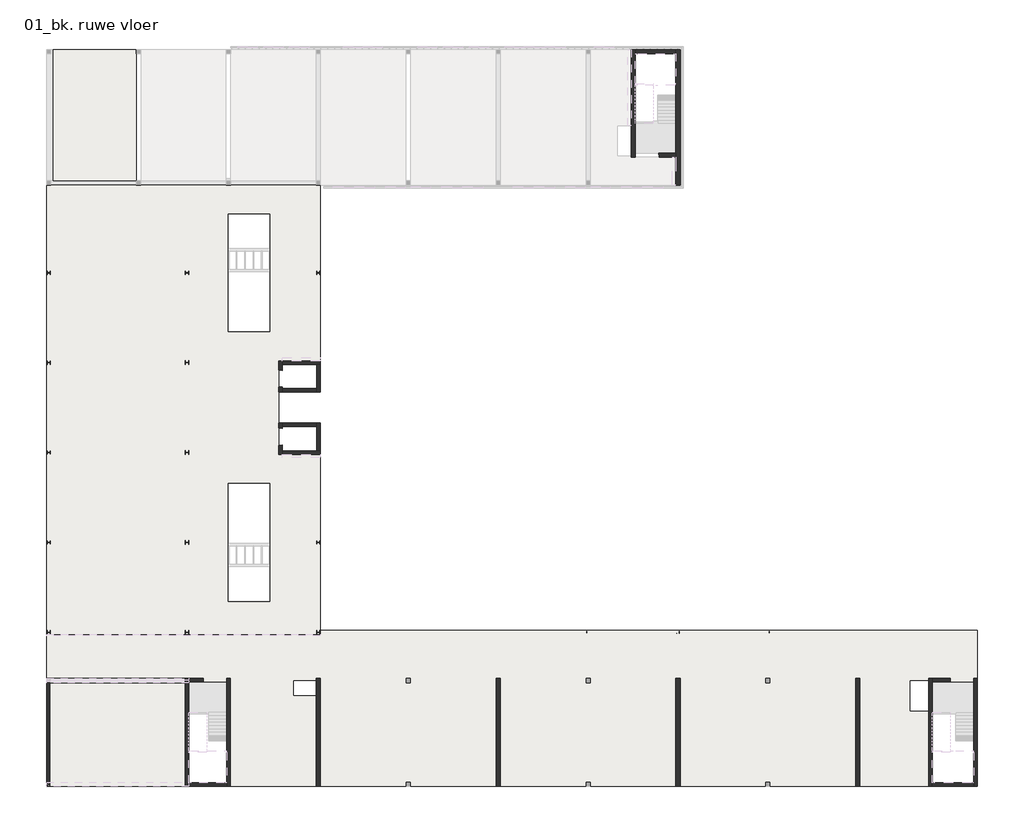
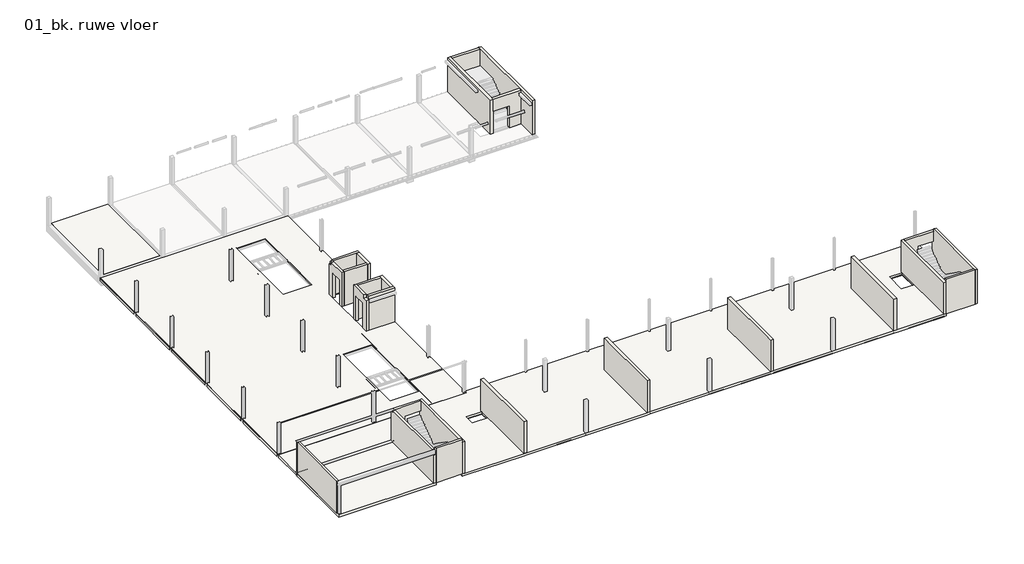
# One storey, part 1 of 4: 25 walls, 20 slabs.
# Revit data of these elements (continued)
# Type "NLRS_21_WA_beton ihw 250_gen_rsf"
#   Keynote = ""
#   Type IfcGUID = "1pBmRfcsbA7BE9s_rekBP3"
#   Description = "buitenwand beton ihw, generiek"
#   Assembly Code = "21.21"
#   IfcExportAs = "IfcWall"
#   Layers, outside or top first: 250 mm "NLRS_f2_beton ihwg_gen_rsf" (function 1)
# Type "NLRS_21_WA_kalkzandsteen CS12 214_gen_rsf"
#   Keynote = ""
#   Type IfcGUID = "2$hNzCXOT3YR8V$0Cfyzq0"
#   Type Comments = "blokken/elementen gelijmd, d =214mm"
#   Description = "dragende buitenwand kalkzandsteen, klasse CS12"
#   Assembly Code = "21.21"
#   IfcExportAs = "IfcWall"
#   Layers, outside or top first: 214 mm "NLRS_f1_kalkzandsteen_gen_rsf" (function 1)
# Type "NLRS_22_WA_beton prefab 300_gen_rsf"
#   Keynote = ""
#   Type IfcGUID = "2ajLwCSRTE_9I1Spg4sCRo"
#   Description = "binnenwand beton prefab, generiek"
#   Assembly Code = "22.21"
#   IfcExportAs = "IfcWall"
#   Layers, outside or top first: 300 mm "NLRS_f2_beton prefab_gen_rsf" (function 1)
# Type "NLRS_21_WA_beton prefab 300_gen_rsf"
#   Keynote = ""
#   Type IfcGUID = "2ajLwCSRTE_9I1Spg4sCru"
#   Description = "buitenwand beton prefab, generiek"
#   Assembly Code = "21.21"
#   IfcExportAs = "IfcWall"
#   Layers, outside or top first: 300 mm "NLRS_f2_beton prefab_gen_rsf" (function 1)
# Type "NLRS_22_WA_beton prefab 250_gen_rsf"
#   Keynote = ""
#   Type IfcGUID = "2GRbcre991teoKeCLB8LsU"
#   Description = "binnenwand beton prefab, generiek"
#   Assembly Code = "22.21"
#   IfcExportAs = "IfcWall"
#   Layers, outside or top first: 250 mm "NLRS_f2_beton prefab_gen_rsf" (function 1)
# Type "NLRS_21_WA_beton prefab 250_gen_rsf"
#   Keynote = ""
#   Type IfcGUID = "3N5NK1g7D9AwpiDnyE93lX"
#   Description = "buitenwand beton prefab, generiek"
#   Assembly Code = "21.21"
#   IfcExportAs = "IfcWall"
#   Layers, outside or top first: 250 mm "NLRS_f2_beton prefab_gen_rsf" (function 1)
# Element 1 (IfcSlab, "NLRS_23_FL_breedplaat 260_gen_rsf")
#   IfcGUID = "2ajLwCSRTE_9I1Spg4tpLw"
#   Comments = ""
#   Height Offset From Level = 0 mm
#   built-in parameter 1001954 = 1
#   IsExternal = no
#   LoadBearing = yes
#   Phase Created = NLRS_nieuw
#   Materials on its faces: "NLRS_f2_beton ihwg_gen_rsf"
# Element 2 (IfcSlab, "NLRS_23_FL_breedplaat 260_gen_rsf")
#   IfcGUID = "3_OCAr9yj6mwah3L5tr_i6"
#   Height Offset From Level = 0 mm
#   built-in parameter 1001954 = 1
#   IsExternal = no
#   LoadBearing = yes
#   Phase Created = NLRS_nieuw
#   Materials on its faces: "NLRS_f2_beton ihwg_gen_rsf"
# Element 3 (IfcSlab, "NLRS_23_FL_druklaag 70_gen_rsf")
#   IfcGUID = "2GRbcre991teoKeCLB8MGT"
#   Height Offset From Level = 0 mm
#   built-in parameter 1001954 = 1
#   IsExternal = no
#   LoadBearing = yes
#   Phase Created = NLRS_nieuw
#   Materials on its faces: "NLRS_f2_beton ihwg_gen_rsf"
# Element 4 (IfcSlab, "NLRS_23_FL_kanaalplaat 260_gen_rsf")
#   IfcGUID = "0zo1UjqZ91lRsfCKsOObA6"
#   built-in parameter 1001955 = -1.5708 (stored number, unit not read)
#   Height Offset From Level = -70 mm
#   built-in parameter 1001954 = 1
#   IsExternal = no
#   LoadBearing = yes
#   Phase Created = NLRS_nieuw
#   Materials on its faces: "NLRS_f2_beton prefab_gen_rsf"
# Element 5 (IfcSlab, "NLRS_23_FL_kanaalplaat 260_gen_rsf")
#   IfcGUID = "0zo1UjqZ91lRsfCKsOObtg"
#   built-in parameter 1001955 = -1.5708 (stored number, unit not read)
#   Height Offset From Level = -70 mm
#   built-in parameter 1001954 = 1
#   IsExternal = no
#   LoadBearing = yes
#   Phase Created = NLRS_nieuw
#   Materials on its faces: "NLRS_f2_beton prefab_gen_rsf"
# Element 6 (IfcSlab, "NLRS_23_FL_kanaalplaat 260_gen_rsf")
#   IfcGUID = "0zo1UjqZ91lRsfCKsOObzx"
#   built-in parameter 1001955 = -1.5708 (stored number, unit not read)
#   Height Offset From Level = -70 mm
#   built-in parameter 1001954 = 1
#   IsExternal = no
#   LoadBearing = yes
#   Phase Created = NLRS_nieuw
#   Materials on its faces: "NLRS_f2_beton prefab_gen_rsf"
# Element 7 (IfcSlab, "NLRS_23_FL_kanaalplaat 260_gen_rsf")
#   IfcGUID = "0OswKhMc1Dju7i6LqsClK9"
#   built-in parameter 1001955 = -1.5708 (stored number, unit not read)
#   Height Offset From Level = -70 mm
#   built-in parameter 1001954 = 1
#   IsExternal = no
#   LoadBearing = yes
#   Phase Created = NLRS_nieuw
#   Materials on its faces: "NLRS_f2_beton prefab_gen_rsf"
# Element 8 (IfcSlab, "NLRS_23_FL_kanaalplaat 260_gen_rsf")
#   IfcGUID = "0OswKhMc1Dju7i6LqsClM0"
#   built-in parameter 1001955 = 1.5708 (stored number, unit not read)
#   Height Offset From Level = -70 mm
#   built-in parameter 1001954 = 1
#   IsExternal = no
#   LoadBearing = yes
#   Phase Created = NLRS_nieuw
#   Materials on its faces: "NLRS_f2_beton prefab_gen_rsf"
# Element 9 (IfcSlab, "NLRS_23_FL_kanaalplaat 260_gen_rsf")
#   IfcGUID = "0OswKhMc1Dju7i6LqsClMb"
#   Height Offset From Level = -70 mm
#   built-in parameter 1001954 = 1
#   IsExternal = no
#   LoadBearing = yes
#   Phase Created = NLRS_nieuw
#   Materials on its faces: "NLRS_f2_beton prefab_gen_rsf"
# Element 10 (IfcSlab, "NLRS_23_FL_kanaalplaat 260_gen_rsf")
#   IfcGUID = "0OswKhMc1Dju7i6LqsClTA"
#   built-in parameter 1001955 = -1.5708 (stored number, unit not read)
#   Height Offset From Level = -70 mm
#   built-in parameter 1001954 = 1
#   IsExternal = no
#   LoadBearing = yes
#   Phase Created = NLRS_nieuw
#   Materials on its faces: "NLRS_f2_beton prefab_gen_rsf"
# Element 11 (IfcSlab, "NLRS_23_FL_kanaalplaat 260_gen_rsf")
#   IfcGUID = "0OswKhMc1Dju7i6LqsCl1Q"
#   built-in parameter 1001955 = 1.5708 (stored number, unit not read)
#   Height Offset From Level = -70 mm
#   built-in parameter 1001954 = 1
#   IsExternal = no
#   LoadBearing = yes
#   Phase Created = NLRS_nieuw
#   Materials on its faces: "NLRS_f2_beton prefab_gen_rsf"
# Element 12 (IfcSlab, "NLRS_23_FL_kanaalplaat 260_gen_rsf")
#   IfcGUID = "0OswKhMc1Dju7i6LqsCl1J"
#   built-in parameter 1001955 = 1.5708 (stored number, unit not read)
#   Height Offset From Level = -70 mm
#   built-in parameter 1001954 = 1
#   IsExternal = no
#   LoadBearing = yes
#   Phase Created = NLRS_nieuw
#   Materials on its faces: "NLRS_f2_beton prefab_gen_rsf"
# Element 13 (IfcSlab, "NLRS_23_FL_kanaalplaat 260_gen_rsf")
#   IfcGUID = "0OswKhMc1Dju7i6LqsCl1k"
#   built-in parameter 1001955 = 1.5708 (stored number, unit not read)
#   Height Offset From Level = -70 mm
#   built-in parameter 1001954 = 1
#   IsExternal = no
#   LoadBearing = yes
#   Phase Created = NLRS_nieuw
#   Materials on its faces: "NLRS_f2_beton prefab_gen_rsf"
# Element 14 (IfcSlab, "NLRS_23_FL_kanaalplaat 260_gen_rsf")
#   IfcGUID = "0OswKhMc1Dju7i6LqsCl1d"
#   built-in parameter 1001955 = -1.5708 (stored number, unit not read)
#   Height Offset From Level = -70 mm
#   built-in parameter 1001954 = 1
#   IsExternal = no
#   LoadBearing = yes
#   Phase Created = NLRS_nieuw
#   Materials on its faces: "NLRS_f2_beton prefab_gen_rsf"
# Element 15 (IfcSlab, "NLRS_23_FL_kanaalplaat 260_gen_rsf")
#   IfcGUID = "0OswKhMc1Dju7i6LqsCl1m"
#   Height Offset From Level = -70 mm
#   built-in parameter 1001954 = 1
#   IsExternal = no
#   LoadBearing = yes
#   Phase Created = NLRS_nieuw
#   Materials on its faces: "NLRS_f2_beton prefab_gen_rsf"
# Element 16 (IfcSlab, "NLRS_23_FL_kanaalplaat 260_gen_rsf")
#   IfcGUID = "0OswKhMc1Dju7i6LqsCl2B"
#   built-in parameter 1001955 = 1.5708 (stored number, unit not read)
#   Height Offset From Level = -70 mm
#   built-in parameter 1001954 = 1
#   IsExternal = no
#   LoadBearing = yes
#   Phase Created = NLRS_nieuw
#   Materials on its faces: "NLRS_f2_beton prefab_gen_rsf"
# Element 17 (IfcSlab, "NLRS_23_FL_breedplaat 260_gen_rsf")
#   IfcGUID = "3aMdMHoe12P9KDGPyaIhcT"
#   built-in parameter 1001955 = 1.5708 (stored number, unit not read)
#   Height Offset From Level = 0 mm
#   built-in parameter 1001954 = 1
#   IsExternal = no
#   LoadBearing = yes
#   Phase Created = NLRS_nieuw
#   Materials on its faces: "NLRS_f2_beton ihwg_gen_rsf"
# Element 18 (IfcSlab, "NLRS_23_FL_breedplaat schil 60_gen_rsf")
#   IfcGUID = "2hjDq_lp57$vrUvPCETdlA"
#   Comments = ""
#   built-in parameter 1001955 = -1.5708 (stored number, unit not read)
#   Height Offset From Level = -200 mm
#   built-in parameter 1001954 = 1
#   IsExternal = no
#   LoadBearing = yes
#   Phase Created = NLRS_nieuw
#   Materials on its faces: "NLRS_f2_beton prefab_gen_rsf"
# Element 19 (IfcSlab, "NLRS_23_FL_breedplaat schil 60_gen_rsf")
#   IfcGUID = "2hjDq_lp57$vrUvPCETOIZ"
#   Comments = ""
#   built-in parameter 1001955 = -1.5708 (stored number, unit not read)
#   Height Offset From Level = -200 mm
#   built-in parameter 1001954 = 1
#   IsExternal = no
#   LoadBearing = yes
#   Phase Created = NLRS_nieuw
#   Materials on its faces: "NLRS_f2_beton prefab_gen_rsf"
# Element 20 (IfcSlab, "NLRS_23_FL_breedplaat schil 60_gen_rsf")
#   IfcGUID = "1q3Kx8wcTFnf_3PJz4ij95"
#   Comments = ""
#   Height Offset From Level = -200 mm
#   built-in parameter 1001954 = 1
#   IsExternal = no
#   LoadBearing = yes
#   Phase Created = NLRS_nieuw
#   Materials on its faces: "NLRS_f2_beton prefab_gen_rsf"
# Element 21 (IfcWall, "NLRS_22_WA_beton ihw 250_gen_rsf")
#   IfcGUID = "13lTCcCQ95UOWcvnmPh7qn"
#   Comments = ""
#   Top Offset = 0 mm
#   Base Offset = 0 mm
#   wall height = 3540 mm
#   IsExternal = no
#   LoadBearing = yes
#   Phase Created = NLRS_nieuw
#   Base Constraint = 01_bk. ruwe vloer
#   Top Constraint = 02_ok ruwe vloer
#   Materials on its faces: "NLRS_f2_beton ihwg_gen_rsf"
# Element 22 (IfcWall, "NLRS_22_WA_beton ihw 250_gen_rsf")
#   IfcGUID = "13lTCcCQ95UOWcvnmPh7qi"
#   Comments = ""
#   Top Offset = 0 mm
#   Base Offset = 0 mm
#   wall height = 3540 mm
#   IsExternal = no
#   LoadBearing = yes
#   Phase Created = NLRS_nieuw
#   Base Constraint = 01_bk. ruwe vloer
#   Top Constraint = 02_ok ruwe vloer
#   Materials on its faces: "NLRS_f2_beton ihwg_gen_rsf"
# Element 23 (IfcWall, "NLRS_22_WA_beton ihw 300_gen_rsf")
#   IfcGUID = "13lTCcCQ95UOWcvnmPh7qk"
#   Comments = ""
#   Top Offset = 0 mm
#   Base Offset = 0 mm
#   wall height = 3540 mm
#   IsExternal = no
#   LoadBearing = yes
#   Phase Created = NLRS_nieuw
#   Base Constraint = 01_bk. ruwe vloer
#   Top Constraint = 02_ok ruwe vloer
#   Materials on its faces: "NLRS_f2_beton ihwg_gen_rsf"
# Element 24 (IfcWall, "NLRS_22_WA_beton ihw 300_gen_rsf")
#   IfcGUID = "13lTCcCQ95UOWcvnmPh7qg"
#   Comments = ""
#   Top Offset = 0 mm
#   Base Offset = 0 mm
#   wall height = 3540 mm
#   IsExternal = no
#   LoadBearing = yes
#   Phase Created = NLRS_nieuw
#   Base Constraint = 01_bk. ruwe vloer
#   Top Constraint = 02_ok ruwe vloer
#   Materials on its faces: "NLRS_f2_beton ihwg_gen_rsf"
# Element 25 (IfcWall, "NLRS_22_WA_beton ihw 300_gen_rsf")
#   IfcGUID = "13lTCcCQ95UOWcvnmPh7qc"
#   Comments = ""
#   Top Offset = 0 mm
#   Base Offset = 0 mm
#   wall height = 3540 mm
#   IsExternal = no
#   LoadBearing = yes
#   Phase Created = NLRS_nieuw
#   Base Constraint = 01_bk. ruwe vloer
#   Top Constraint = 02_ok ruwe vloer
#   Materials on its faces: "NLRS_f2_beton ihwg_gen_rsf"
# Element 26 (IfcWall, "NLRS_22_WA_beton ihw 300_gen_rsf")
#   IfcGUID = "13lTCcCQ95UOWcvnmPh7qY"
#   Comments = ""
#   Top Offset = 0 mm
#   Base Offset = 0 mm
#   wall height = 3540 mm
#   IsExternal = no
#   LoadBearing = yes
#   Phase Created = NLRS_nieuw
#   Base Constraint = 01_bk. ruwe vloer
#   Top Constraint = 02_ok ruwe vloer
#   Materials on its faces: "NLRS_f2_beton ihwg_gen_rsf"
# Element 27 (IfcWall, "NLRS_21_WA_beton ihw 250_gen_rsf")
#   IfcGUID = "13lTCcCQ95UOWcvnmPh7rS"
#   Comments = ""
#   Top Offset = 0 mm
#   Base Offset = 0 mm
#   wall height = 3800 mm
#   IsExternal = yes
#   LoadBearing = yes
#   Phase Created = NLRS_nieuw
#   Base Constraint = 01_bk. ruwe vloer
#   Top Constraint = 02_bk ruwe vloer
#   Materials on its faces: "NLRS_f2_beton ihwg_gen_rsf"
# Element 28 (IfcWall, "NLRS_21_WA_kalkzandsteen CS12 214_gen_rsf")
#   IfcGUID = "13lTCcCQ95UOWcvnmPh7rU"
#   Comments = ""
#   Top Offset = 0 mm
#   Base Offset = 0 mm
#   wall height = 3540 mm
#   IsExternal = yes
#   LoadBearing = yes
#   Phase Created = NLRS_nieuw
#   Base Constraint = 01_bk. ruwe vloer
#   Top Constraint = 02_ok ruwe vloer
#   Materials on its faces: "NLRS_f1_kalkzandsteen_gen_rsf"
# Element 29 (IfcWall, "NLRS_21_WA_beton ihw 250_gen_rsf")
#   IfcGUID = "13lTCcCQ95UOWcvnmPh7rO"
#   Top Offset = 0 mm
#   Base Offset = 0 mm
#   wall height = 3800 mm
#   IsExternal = yes
#   LoadBearing = yes
#   Phase Created = NLRS_nieuw
#   Base Constraint = 01_bk. ruwe vloer
#   Top Constraint = 02_bk ruwe vloer
#   Materials on its faces: "NLRS_f2_beton ihwg_gen_rsf"
# Element 30 (IfcWall, "NLRS_22_WA_beton ihw 250_gen_rsf")
#   IfcGUID = "13lTCcCQ95UOWcvnmPh7rQ"
#   Top Offset = 0 mm
#   Base Offset = 0 mm
#   wall height = 3540 mm
#   IsExternal = no
#   LoadBearing = yes
#   Phase Created = NLRS_nieuw
#   Base Constraint = 01_bk. ruwe vloer
#   Top Constraint = 02_ok ruwe vloer
#   Materials on its faces: "NLRS_f2_beton ihwg_gen_rsf"
# Element 31 (IfcWall, "NLRS_22_WA_beton ihw 250_gen_rsf")
#   IfcGUID = "13lTCcCQ95UOWcvnmPh7rK"
#   Comments = ""
#   Top Offset = 0 mm
#   Base Offset = 0 mm
#   wall height = 3540 mm
#   IsExternal = no
#   LoadBearing = yes
#   Phase Created = NLRS_nieuw
#   Base Constraint = 01_bk. ruwe vloer
#   Top Constraint = 02_ok ruwe vloer
#   Materials on its faces: "NLRS_f2_beton ihwg_gen_rsf"
# Element 32 (IfcWall, "NLRS_21_WA_beton ihw 250_gen_rsf")
#   IfcGUID = "13lTCcCQ95UOWcvnmPh7rM"
#   Top Offset = 0 mm
#   Base Offset = 0 mm
#   wall height = 3800 mm
#   IsExternal = yes
#   LoadBearing = yes
#   Phase Created = NLRS_nieuw
#   Base Constraint = 01_bk. ruwe vloer
#   Top Constraint = 02_bk ruwe vloer
#   Materials on its faces: "NLRS_f2_beton ihwg_gen_rsf"
# Element 33 (IfcWall, "NLRS_22_WA_beton ihw 250_gen_rsf")
#   IfcGUID = "13lTCcCQ95UOWcvnmPh7rG"
#   Top Offset = 0 mm
#   Base Offset = 0 mm
#   wall height = 3540 mm
#   IsExternal = no
#   LoadBearing = yes
#   Phase Created = NLRS_nieuw
#   Base Constraint = 01_bk. ruwe vloer
#   Top Constraint = 02_ok ruwe vloer
#   Materials on its faces: "NLRS_f2_beton ihwg_gen_rsf"
# Element 34 (IfcWall, "NLRS_22_WA_beton prefab 300_gen_rsf")
#   IfcGUID = "13lTCcCQ95UOWcvnmPh7s_"
#   Comments = ""
#   built-in parameter 1001111 = 20 mm
#   Top Offset = 0 mm
#   Base Offset = 20 mm
#   wall height = 3780 mm
#   IsExternal = no
#   LoadBearing = yes
#   Phase Created = NLRS_nieuw
#   Base Constraint = 01_bk. ruwe vloer
#   Top Constraint = 02_bk ruwe vloer
#   Materials on its faces: "NLRS_f2_beton prefab_gen_rsf"
# Element 35 (IfcWall, "NLRS_21_WA_beton prefab 300_gen_rsf")
#   IfcGUID = "13lTCcCQ95UOWcvnmPh7sx"
#   Comments = ""
#   built-in parameter 1001111 = 20 mm
#   Top Offset = 0 mm
#   Base Offset = 20 mm
#   wall height = 3780 mm
#   IsExternal = yes
#   LoadBearing = yes
#   Phase Created = NLRS_nieuw
#   Base Constraint = 01_bk. ruwe vloer
#   Top Constraint = 02_bk ruwe vloer
#   Materials on its faces: "NLRS_f2_beton prefab_gen_rsf"
# Element 36 (IfcWall, "NLRS_21_WA_beton prefab 300_gen_rsf")
#   IfcGUID = "13lTCcCQ95UOWcvnmPh7sr"
#   Comments = ""
#   built-in parameter 1001111 = 20 mm
#   Top Offset = 0 mm
#   Base Offset = 20 mm
#   wall height = 3780 mm
#   IsExternal = yes
#   LoadBearing = yes
#   Phase Created = NLRS_nieuw
#   Base Constraint = 01_bk. ruwe vloer
#   Top Constraint = 02_bk ruwe vloer
#   Materials on its faces: "NLRS_f2_beton prefab_gen_rsf"
# Element 37 (IfcWall, "NLRS_22_WA_beton prefab 300_gen_rsf")
#   IfcGUID = "13lTCcCQ95UOWcvnmPh7st"
#   Comments = ""
#   built-in parameter 1001111 = 20 mm
#   Top Offset = 0 mm
#   Base Offset = 20 mm
#   wall height = 3780 mm
#   IsExternal = no
#   LoadBearing = yes
#   Phase Created = NLRS_nieuw
#   Base Constraint = 01_bk. ruwe vloer
#   Top Constraint = 02_bk ruwe vloer
#   Materials on its faces: "NLRS_f2_beton prefab_gen_rsf"
# Element 38 (IfcWall, "NLRS_22_WA_beton prefab 250_gen_rsf")
#   IfcGUID = "13lTCcCQ95UOWcvnmPh7uI"
#   built-in parameter 1001111 = 20 mm
#   Top Offset = 0 mm
#   Base Offset = 20 mm
#   wall height = 3780 mm
#   IsExternal = no
#   LoadBearing = yes
#   Phase Created = NLRS_nieuw
#   Base Constraint = 01_bk. ruwe vloer
#   Top Constraint = 02_bk ruwe vloer
#   Materials on its faces: "NLRS_f2_beton prefab_gen_rsf"
# Element 39 (IfcWall, "NLRS_22_WA_beton prefab 250_gen_rsf")
#   IfcGUID = "13lTCcCQ95UOWcvnmPh7uC"
#   built-in parameter 1001111 = 20 mm
#   Top Offset = 0 mm
#   Base Offset = 20 mm
#   wall height = 3780 mm
#   IsExternal = no
#   LoadBearing = yes
#   Phase Created = NLRS_nieuw
#   Base Constraint = 01_bk. ruwe vloer
#   Top Constraint = 02_bk ruwe vloer
#   Materials on its faces: "NLRS_f2_beton prefab_gen_rsf"
# Element 40 (IfcWall, "NLRS_22_WA_beton prefab 250_gen_rsf")
#   IfcGUID = "13lTCcCQ95UOWcvnmPh7uE"
#   built-in parameter 1001111 = 20 mm
#   Top Offset = 0 mm
#   Base Offset = 20 mm
#   wall height = 3780 mm
#   IsExternal = no
#   LoadBearing = yes
#   Phase Created = NLRS_nieuw
#   Base Constraint = 01_bk. ruwe vloer
#   Top Constraint = 02_bk ruwe vloer
#   Materials on its faces: "NLRS_f2_beton prefab_gen_rsf"
# Element 41 (IfcWall, "NLRS_21_WA_beton prefab 250_gen_rsf")
#   IfcGUID = "13lTCcCQ95UOWcvnmPh7u8"
#   built-in parameter 1001111 = 20 mm
#   Top Offset = 0 mm
#   Base Offset = 20 mm
#   wall height = 3780 mm
#   IsExternal = yes
#   LoadBearing = yes
#   Phase Created = NLRS_nieuw
#   Base Constraint = 01_bk. ruwe vloer
#   Top Constraint = 02_bk ruwe vloer
#   Materials on its faces: "NLRS_f2_beton prefab_gen_rsf"
# Element 42 (IfcWall, "NLRS_22_WA_beton prefab 250_gen_rsf")
#   IfcGUID = "13lTCcCQ95UOWcvnmPh7uA"
#   built-in parameter 1001111 = 20 mm
#   Top Offset = 0 mm
#   Base Offset = 20 mm
#   wall height = 3780 mm
#   IsExternal = no
#   LoadBearing = yes
#   Phase Created = NLRS_nieuw
#   Base Constraint = 01_bk. ruwe vloer
#   Top Constraint = 02_bk ruwe vloer
#   Materials on its faces: "NLRS_f2_beton prefab_gen_rsf"
# Element 43 (IfcWall, "NLRS_22_WA_beton prefab 250_gen_rsf")
#   IfcGUID = "13lTCcCQ95UOWcvnmPh7u4"
#   built-in parameter 1001111 = 20 mm
#   Top Offset = 0 mm
#   Base Offset = 20 mm
#   wall height = 3780 mm
#   IsExternal = no
#   LoadBearing = yes
#   Phase Created = NLRS_nieuw
#   Base Constraint = 01_bk. ruwe vloer
#   Top Constraint = 02_bk ruwe vloer
#   Materials on its faces: "NLRS_f2_beton prefab_gen_rsf"
# Element 44 (IfcWall, "NLRS_22_WA_beton prefab 250_gen_rsf")
#   IfcGUID = "13lTCcCQ95UOWcvnmPh7u6"
#   built-in parameter 1001111 = 20 mm
#   Top Offset = 0 mm
#   Base Offset = 20 mm
#   wall height = 3780 mm
#   IsExternal = no
#   LoadBearing = yes
#   Phase Created = NLRS_nieuw
#   Base Constraint = 01_bk. ruwe vloer
#   Top Constraint = 02_bk ruwe vloer
#   Materials on its faces: "NLRS_f2_beton prefab_gen_rsf"
# Element 45 (IfcWall, "NLRS_21_WA_beton prefab 250_gen_rsf")
#   IfcGUID = "13lTCcCQ95UOWcvnmPh7u0"
#   built-in parameter 1001111 = 20 mm
#   Top Offset = 0 mm
#   Base Offset = 20 mm
#   wall height = 3780 mm
#   IsExternal = yes
#   LoadBearing = yes
#   Phase Created = NLRS_nieuw
#   Base Constraint = 01_bk. ruwe vloer
#   Top Constraint = 02_bk ruwe vloer
#   Materials on its faces: "NLRS_f2_beton prefab_gen_rsf"
# Materials
#   "NLRS_f2_beton ihwg_gen_rsf": class "F - Niet gebakken kunststeen", colour RGB 129 133 118, transparency 0, Keynote = "f2", Manufacturer = "Revit Standards Foundation", URL = "www.revitstandards.org", Description = "beton ihwg", Cost = 0
#   "NLRS_f2_beton prefab_gen_rsf": class "F - Niet gebakken kunststeen", colour RGB 129 133 118, transparency 0, Keynote = "f2", Manufacturer = "Revit Standards Foundation", URL = "www.revitstandards.org", Description = "beton prefab", Cost = 0
#   "NLRS_f1_kalkzandsteen_gen_rsf": class "F - Niet gebakken kunststeen", colour RGB 223 221 219, transparency 0, Keynote = "f1", Manufacturer = "Revit Standards Foundation", URL = "www.revitstandards.org", Description = "kalkzandsteen", Cost = 0
